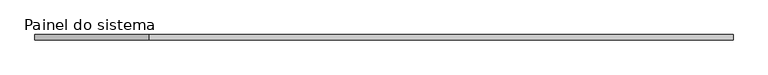
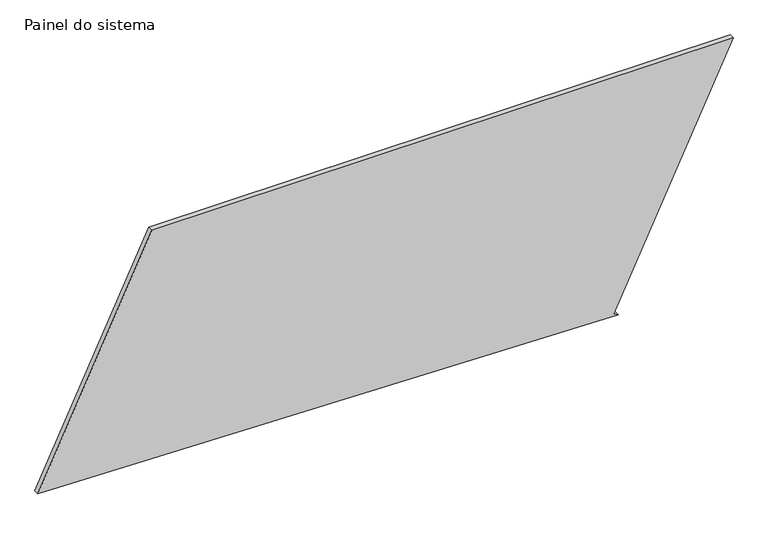
"""IFC4 building model written with IfcOpenShell, lengths in millimetres: plate geometry, Painel do sistema : Envidraçado."""

from ifc_helpers import new_model, si_unit, frame, origin, place, context, project, spatial, polyline, outline, extrude, source, transform, mapped, element, save


def painel_do_sistema_d6e497bb(model_context):
    return source(origin(), model_context, "Body", "SweptSolid", [
        extrude(outline(polyline([(0.0, 1130.7690534), (10.7698497, 1108.2077959), (1225.1878303, 1687.9227829), (1225.1878303, -1135.0902487), (67.0846505, -1687.9227829), (0.0, 1130.7690534)])), frame((0.0, 24.5, 0.0), z_axis=(0.0, 1.0, 0.0), x_axis=(0.0, 0.0, 1.0)), (0.0, 0.0, 1.0), 25.0),
    ])


if __name__ == "__main__":
    model = new_model("IFC4")
    model_context = context("Model", 3, world=origin())
    ifc_project = project(units=[si_unit("LENGTHUNIT", "METRE", prefix="MILLI")], contexts=[model_context])
    site = spatial("IfcSite", under=ifc_project)
    building = spatial("IfcBuilding", under=site)
    placement = place(None, origin())
    painel_do_sistema_shape = painel_do_sistema_d6e497bb(model_context)
    element("IfcPlate", 1, ObjectType="Painel do sistema : Envidraçado", at=placement, inside=building, context=model_context, shape_type="MappedRepresentation", body=[
        mapped(painel_do_sistema_shape, transform((0.0, 0.0, 0.0), x_axis=(1.0, 0.0, 0.0), y_axis=(0.0, 1.0, 0.0), z_axis=(0.0, 0.0, 1.0))),
    ])
    save(model, "model.ifc")

# Revit data of these elements
# Type "Painel do sistema : Envidraçado"
#   Construction Type Id = "GSP4R"
#   Analytic Construction = "Vidraça única Pilkington 1/8 pol"
#   Visual Light Transmittance = 0.9
#   Solar Heat Gain Coefficient = 0.86
#   Heat Transfer Coefficient (U) = 6.7069 W/(m²·K)
# Element 1 (IfcPlate, "Painel do sistema : Envidraçado")
#   Materials on its faces: "Vidro"
# Materials
#   "Vidro": class "Vidro", colour RGB 0 128 192, transparency 0.9, Description = "Vidro de sílica", Cost = 0
